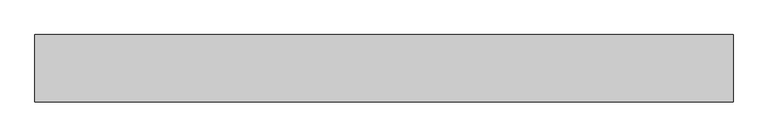
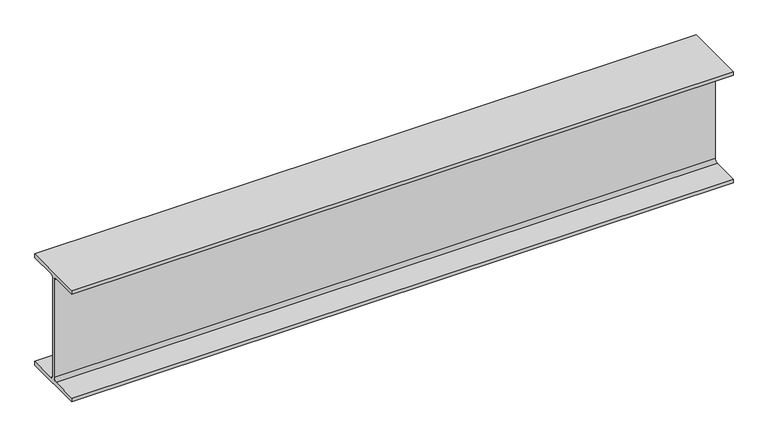
"""IFC4 building model written with IfcOpenShell, lengths in millimetres: beam geometry, Old_Steel Beam_H-KSD3502 : H_SB_ASB_H-200×200x8x12."""

import ifcopenshell
import ifcopenshell.guid

model = None  # the IFC model being written
_history = None  # IfcOwnerHistory: only IFC2X3 demands one
_inside = {}  # id of a spatial element -> (the spatial element, [elements in it])
_under = {}  # id of a project, library or spatial element -> (it, [spatial elements below it])
_declared = {}  # id of a project -> (the project, [libraries it declares])
_typed = {}  # id of a type object -> (the type object, [elements of that type])
_made_of = {}  # id of a material, layer set ... -> (it, [elements and type objects made of it])


def new_model(schema):
    """Start an empty IFC model of exactly this schema.

    Asked for "IFC4X3", IfcOpenShell would pick the latest addendum, in which some entities
    have other attributes; the version numbers below select the first issue.
    IFC2X3 requires an IfcOwnerHistory on every rooted entity: one is made here for all.
    """
    global model, _history
    if schema == "IFC4X3":
        model = ifcopenshell.file(schema_version=(4, 3, 0, 0))
    else:
        model = ifcopenshell.file(schema=schema)
    _inside.clear()
    _under.clear()
    _declared.clear()
    _typed.clear()
    _made_of.clear()
    _history = None
    if model.schema == "IFC2X3":
        org = make("IfcOrganization", Name="unknown")
        user = make(
            "IfcPersonAndOrganization",
            ThePerson=make("IfcPerson", FamilyName="unknown"),
            TheOrganization=org,
        )
        app = make(
            "IfcApplication",
            ApplicationDeveloper=org,
            Version="unknown",
            ApplicationFullName="unknown",
            ApplicationIdentifier="unknown",
        )
        _history = make(
            "IfcOwnerHistory",
            OwningUser=user,
            OwningApplication=app,
            ChangeAction="ADDED",
            CreationDate=0,
        )
    return model


def make(cls, **values):
    """One entity of the class cls with the attributes given. An attribute that is None is left unset."""
    return model.create_entity(
        cls, **{name: value for name, value in values.items() if value is not None}
    )


def rooted(cls, **values):
    """An entity with a GlobalId (a new one), such as an element, a storey or a relation."""
    return make(cls, GlobalId=ifcopenshell.guid.new(), OwnerHistory=_history, **values)


def si_unit(unit_type, name, prefix=None):
    """IfcSIUnit, for example si_unit("LENGTHUNIT", "METRE", prefix="MILLI")."""
    return make("IfcSIUnit", UnitType=unit_type, Prefix=prefix, Name=name)


def assignment(units):
    """IfcUnitAssignment: the units of a project."""
    return None if units is None else make("IfcUnitAssignment", Units=units)


def point(xyz):
    """IfcCartesianPoint."""
    return None if xyz is None else make("IfcCartesianPoint", Coordinates=xyz)


def direction(xyz):
    """IfcDirection."""
    return None if xyz is None else make("IfcDirection", DirectionRatios=xyz)


def frame(location, z_axis=None, x_axis=None):
    """IfcAxis2Placement3D, a coordinate frame: its origin and axes. An axis left out is left unset."""
    return make(
        "IfcAxis2Placement3D",
        Location=point(location),
        Axis=direction(z_axis),
        RefDirection=direction(x_axis),
    )


def frame_2d(location, x_axis=None):
    """IfcAxis2Placement2D, a coordinate frame in the plane: its origin and x axis."""
    return make(
        "IfcAxis2Placement2D", Location=point(location), RefDirection=direction(x_axis)
    )


def origin():
    """The frame at (0, 0, 0) with its axes left unset."""
    return frame((0.0, 0.0, 0.0))


def place(relative_to, where):
    """IfcLocalPlacement: puts the frame where relative to a parent placement (None: the world)."""
    return make(
        "IfcLocalPlacement", PlacementRelTo=relative_to, RelativePlacement=where
    )


def context(
    kind, dimensions, precision=None, world=None, true_north=None, identifier=None
):
    """IfcGeometricRepresentationContext, for example the 3D "Model" context."""
    return make(
        "IfcGeometricRepresentationContext",
        ContextIdentifier=identifier,
        ContextType=kind,
        CoordinateSpaceDimension=dimensions,
        Precision=precision,
        WorldCoordinateSystem=world,
        TrueNorth=true_north,
    )


def project(units=None, contexts=None):
    """IfcProject with its units and contexts."""
    return rooted(
        "IfcProject",
        Name="project",
        RepresentationContexts=contexts,
        UnitsInContext=assignment(units),
    )


def spatial(cls, under=None, at=None, **own):
    """A site, building, storey or space (cls), placed at a placement, below another one or the project."""
    s = rooted(cls, ObjectPlacement=at, **own)
    if under is not None:
        _under.setdefault(under.id(), (under, []))[1].append(s)
    return s


def polyline(points):
    """IfcPolyline through the points."""
    return make("IfcPolyline", Points=[point(p) for p in points])


def circle_curve(where, radius):
    """IfcCircle in the frame where."""
    return make("IfcCircle", Position=where, Radius=radius)


def trimmed(basis, trim1, trim2, sense, master):
    """IfcTrimmedCurve: the piece of a basis curve between two trims."""
    return make(
        "IfcTrimmedCurve",
        BasisCurve=basis,
        Trim1=trim1,
        Trim2=trim2,
        SenseAgreement=sense,
        MasterRepresentation=master,
    )


def segment(curve, same_sense, transition):
    """IfcCompositeCurveSegment."""
    return make(
        "IfcCompositeCurveSegment",
        Transition=transition,
        SameSense=same_sense,
        ParentCurve=curve,
    )


def composite_curve(segments, self_intersect=None):
    """IfcCompositeCurve: segments joined end to end."""
    return make("IfcCompositeCurve", Segments=segments, SelfIntersect=self_intersect)


def outline(outer, holes=None, kind="AREA"):
    """IfcArbitraryClosedProfileDef: a profile drawn as a closed curve; with holes, ...WithVoids."""
    if holes is None:
        return make("IfcArbitraryClosedProfileDef", ProfileType=kind, OuterCurve=outer)
    return make(
        "IfcArbitraryProfileDefWithVoids",
        ProfileType=kind,
        OuterCurve=outer,
        InnerCurves=holes,
    )


def extrude(swept, where, along, depth):
    """IfcExtrudedAreaSolid: the profile swept, set in the frame where, extruded along a direction by depth."""
    return make(
        "IfcExtrudedAreaSolid",
        SweptArea=swept,
        Position=where,
        ExtrudedDirection=direction(along),
        Depth=depth,
    )


def shape(context_of_items, identifier, shape_type, items):
    """IfcShapeRepresentation: the items that make up one representation, for example the "Body"."""
    return make(
        "IfcShapeRepresentation",
        ContextOfItems=context_of_items,
        RepresentationIdentifier=identifier,
        RepresentationType=shape_type,
        Items=items,
    )


def source(mapping_origin, context_of_items, identifier, shape_type, items):
    """IfcRepresentationMap: a shape defined once, which mapped items show again and again."""
    return make(
        "IfcRepresentationMap",
        MappingOrigin=mapping_origin,
        MappedRepresentation=shape(context_of_items, identifier, shape_type, items),
    )


def transform(
    local_origin,
    x_axis=None,
    y_axis=None,
    z_axis=None,
    scale=None,
    scale2=None,
    scale3=None,
    uniform=True,
):
    """IfcCartesianTransformationOperator3D, or its non-uniform kind. x_axis, y_axis, z_axis: its Axis1, 2, 3."""
    if uniform:
        return make(
            "IfcCartesianTransformationOperator3D",
            Axis1=direction(x_axis),
            Axis2=direction(y_axis),
            LocalOrigin=point(local_origin),
            Scale=scale,
            Axis3=direction(z_axis),
        )
    return make(
        "IfcCartesianTransformationOperator3DnonUniform",
        Axis1=direction(x_axis),
        Axis2=direction(y_axis),
        LocalOrigin=point(local_origin),
        Scale=scale,
        Axis3=direction(z_axis),
        Scale2=scale2,
        Scale3=scale3,
    )


def mapped(mapping_source, mapping_target):
    """IfcMappedItem: shows the shape of a source again, moved by a transform."""
    return make(
        "IfcMappedItem", MappingSource=mapping_source, MappingTarget=mapping_target
    )


def made_of(thing, what):
    """Note that an element or type object is made of a material, layer set ...; save() writes the relation."""
    if what is not None:
        _made_of.setdefault(what.id(), (what, []))[1].append(thing)
    return thing


def element(
    cls,
    number,
    at=None,
    inside=None,
    cuts=None,
    type_object=None,
    material=None,
    context=None,
    identifier="Body",
    shape_type=None,
    held_by="IfcProductDefinitionShape",
    body=None,
    shapes=None,
    **own,
):
    """One element of the class cls, such as IfcWall. Its Tag is "e" and its number.

    at: its placement. inside: the storey or other place that contains it. cuts: it is an
    opening in that element (IfcRelVoidsElement). A single representation is given by context,
    identifier, shape_type and body (its items); several are given by shapes. held_by: the class
    of the entity that holds the representations. save() writes the other relations.
    """
    e = rooted(cls, Tag="e%d" % number, ObjectPlacement=at, **own)
    if body is not None:
        shapes = [shape(context, identifier, shape_type, body)]
    if shapes is not None:
        e.Representation = make(held_by, Representations=shapes)
    if inside is not None:
        _inside.setdefault(inside.id(), (inside, []))[1].append(e)
    if cuts is not None:
        rooted(
            "IfcRelVoidsElement", RelatingBuildingElement=cuts, RelatedOpeningElement=e
        )
    if type_object is not None:
        _typed.setdefault(type_object.id(), (type_object, []))[1].append(e)
    return made_of(e, material)


def aggregate(whole, parts):
    """IfcRelAggregates: a whole, such as a stair, and the parts it consists of."""
    return rooted("IfcRelAggregates", RelatingObject=whole, RelatedObjects=parts)


def save(model, path):
    """Write the relations noted so far, then the file.

    IfcRelAggregates (storeys below a building ...), IfcRelContainedInSpatialStructure (elements
    in a storey), IfcRelDefinesByType, IfcRelAssociatesMaterial and IfcRelDeclares: one each for
    every whole, place, type object, material and project.
    """
    for whole, parts in _under.values():
        aggregate(whole, parts)
    for where, things in _inside.values():
        rooted(
            "IfcRelContainedInSpatialStructure",
            RelatedElements=things,
            RelatingStructure=where,
        )
    for kind, things in _typed.values():
        rooted("IfcRelDefinesByType", RelatedObjects=things, RelatingType=kind)
    for what, things in _made_of.values():
        rooted("IfcRelAssociatesMaterial", RelatedObjects=things, RelatingMaterial=what)
    for by, libraries in _declared.values():
        rooted("IfcRelDeclares", RelatingContext=by, RelatedDefinitions=libraries)
    model.write(path)


def beam_c4b8d585(model_context):
    return source(origin(), model_context, "Body", "SweptSolid", [
        extrude(outline(composite_curve([segment(polyline([(82.5, -141.5), (82.5, -151.7), (-82.5, -151.7), (-82.5, -141.5), (-11.9, -141.5)]), True, "CONTINUOUS"), segment(trimmed(circle_curve(frame_2d((-11.9, -132.6)), 8.9), [point((-11.9, -141.5))], [point((-3.0, -132.6))], True, "CARTESIAN"), True, "CONTINUOUS"), segment(polyline([(-3.0, -132.6), (-3.0, 132.6)]), True, "CONTINUOUS"), segment(trimmed(circle_curve(frame_2d((-11.9, 132.6)), 8.9), [point((-3.0, 132.6))], [point((-11.9, 141.5))], True, "CARTESIAN"), True, "CONTINUOUS"), segment(polyline([(-11.9, 141.5), (-82.5, 141.5), (-82.5, 151.7), (82.5, 151.7), (82.5, 141.5), (11.9, 141.5)]), True, "CONTINUOUS"), segment(trimmed(circle_curve(frame_2d((11.9, 132.6)), 8.9), [point((11.9, 141.5))], [point((3.0, 132.6))], True, "CARTESIAN"), True, "CONTINUOUS"), segment(polyline([(3.0, 132.6), (3.0, -132.6)]), True, "CONTINUOUS"), segment(trimmed(circle_curve(frame_2d((11.9, -132.6)), 8.9), [point((3.0, -132.6))], [point((11.9, -141.5))], True, "CARTESIAN"), True, "CONTINUOUS"), segment(polyline([(11.9, -141.5), (82.5, -141.5)]), True, "CONTINUOUS")], self_intersect=False)), frame((-969.5119577, 0.0, 0.0), z_axis=(1.0, 0.0, 0.0), x_axis=(0.0, 1.0, 0.0)), (0.0, 0.0, 1.0), 1706.6963833),
    ])


if __name__ == "__main__":
    model = new_model("IFC4")
    model_context = context("Model", 3, world=origin())
    ifc_project = project(units=[si_unit("LENGTHUNIT", "METRE", prefix="MILLI")], contexts=[model_context])
    site = spatial("IfcSite", under=ifc_project)
    building = spatial("IfcBuilding", under=site)
    placement = place(None, origin())
    beam_shape = beam_c4b8d585(model_context)
    element("IfcBeam", 1, ObjectType="Old_Steel Beam_H-KSD3502 : H_SB_ASB_H-200×200x8x12", at=placement, inside=building, context=model_context, shape_type="MappedRepresentation", body=[
        mapped(beam_shape, transform((0.0, 0.0, 0.0), x_axis=(1.0, 0.0, 0.0), y_axis=(0.0, 1.0, 0.0), z_axis=(0.0, 0.0, 1.0))),
    ])
    save(model, "model.ifc")

# Revit data of these elements
# Type "Old_Steel Beam_H-KSD3502 : H_SB_ASB_H-200×200x8x12"
#   Width = 20.0 cm
#   Web Thickness = 0.8 cm
#   Web Fillet = 1.3 cm
#   Warping Constant = 141376.0 cm⁶
#   Torsional Moment of Inertia = 26.2485 cm⁴
#   Torsional Modulus = 1.0 cm³
#   Section Area = 63.53 cm²
#   Plastic Modulus weak axis = 244.0 cm³
#   Plastic Modulus strong axis = 525.0 cm³
#   Perimeter = 1.16 m²/m
#   Nominal Weight = 49.90 kgf/m
#   Moment of Inertia weak axis = 1600.00 cm⁴
#   Moment of Inertia strong axis = 4720.00 cm⁴
#   Height = 20.0 cm
#   Flange Thickness = 1.2 cm
#   Elastic Modulus weak axis = 160.0 cm³
#   Elastic Modulus strong axis = 472.0 cm³
#   Centroid Vertical = 10.0 cm
#   Centroid Horizontal = 10.0 cm
#   Length [instance default] = 1.5240 m
#   Structural Material [instance default] = Steel, 45-345
#   Assembly Code = ""
# Element 1 (IfcBeam, "Old_Steel Beam_H-KSD3502 : H_SB_ASB_H-200×200x8x12")
#   Structural Material = none
# Materials
#   "Steel, 45-345": class "Metal", colour RGB 189 187 185, transparency 0, Description = "Steel 345 MPa", Cost = 0
